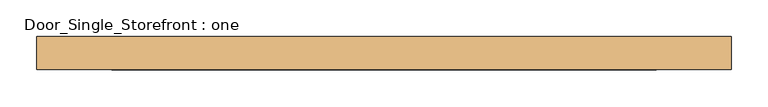
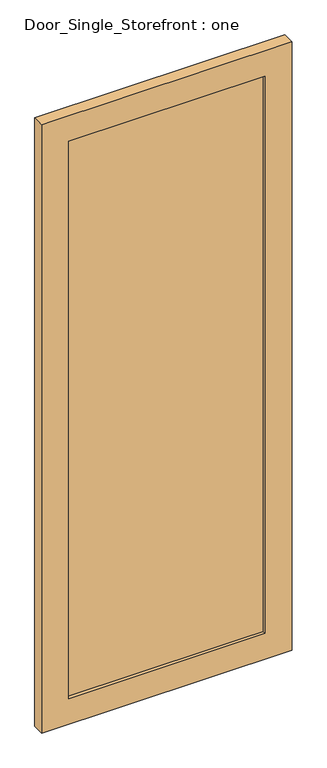
"""IFC4 building model written with IfcOpenShell, lengths in millimetres: door geometry, Door_Single_Storefront : one."""

from ifc_helpers import new_model, si_unit, frame, origin, place, context, project, spatial, polyline, outline, extrude, source, transform, mapped, element, save


def door_single_storefront_one_56ac6ec7(model_context):
    return source(origin(), model_context, "Body", "SweptSolid", [
        extrude(outline(polyline([(368.3, -19.05), (368.3, -38.1), (-368.3, -38.1), (-368.3, -19.05), (368.3, -19.05)])), frame((0.0, 0.0, 101.6), z_axis=(0.0, 0.0, 1.0), x_axis=(1.0, 0.0, 0.0)), (0.0, 0.0, 1.0), 2209.8),
        extrude(outline(polyline([(2413.0, -469.9), (0.0, -469.9), (0.0, 469.9), (2413.0, 469.9), (2413.0, -469.9)]), holes=[polyline([(101.6, 368.3), (101.6, -368.3), (2311.4, -368.3), (2311.4, 368.3), (101.6, 368.3)])]), frame((0.0, -50.8, 0.0), z_axis=(0.0, 1.0, 0.0), x_axis=(0.0, 0.0, 1.0)), (0.0, 0.0, 1.0), 44.45),
    ])


if __name__ == "__main__":
    model = new_model("IFC4")
    model_context = context("Model", 3, world=origin())
    ifc_project = project(units=[si_unit("LENGTHUNIT", "METRE", prefix="MILLI")], contexts=[model_context])
    site = spatial("IfcSite", under=ifc_project)
    building = spatial("IfcBuilding", under=site)
    placement = place(None, origin())
    door_single_storefront_one_shape = door_single_storefront_one_56ac6ec7(model_context)
    element("IfcDoor", 1, ObjectType="Door_Single_Storefront : one", at=placement, inside=building, context=model_context, shape_type="MappedRepresentation", body=[
        mapped(door_single_storefront_one_shape, transform((0.0, 0.0, 0.0), x_axis=(1.0, 0.0, 0.0), y_axis=(0.0, 1.0, 0.0), z_axis=(0.0, 0.0, 1.0))),
    ])
    save(model, "model.ifc")

# Revit data of these elements
# Type "Door_Single_Storefront : one"
#   Type Mark = "27"
#   Analytic Construction = "<None>"
#   Stile_Width = 0' - 4"
#   Door_Thickness = 0' - 1 3/4"
#   Door_Offset = 0' - 2"
#   Glass_Material = Glass
#   Frame_Material = Aluminum
#   Function = (empty or 0)
# Element 1 (IfcDoor, "Door_Single_Storefront : one")
#   Materials on its faces: "Aluminum", "Glass"
# Materials
#   "Glass": class "Glass", colour RGB 0 128 192, transparency 0.75, Description = "Soda Lime Glass", Cost = 0
#   "Aluminum": class "Metal", colour RGB 247 247 247, transparency 0, Description = "Aluminum 6061", Cost = 0
